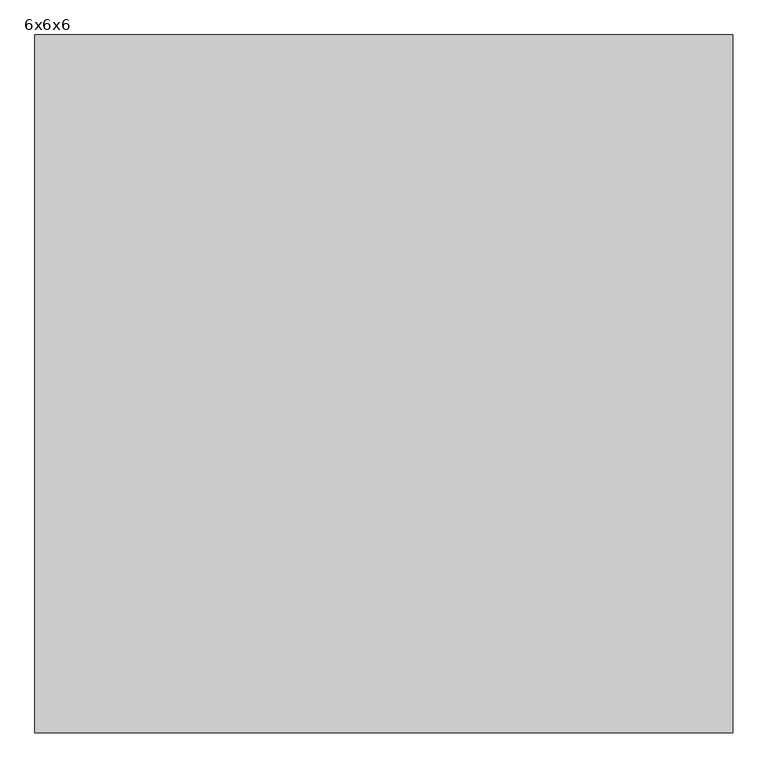
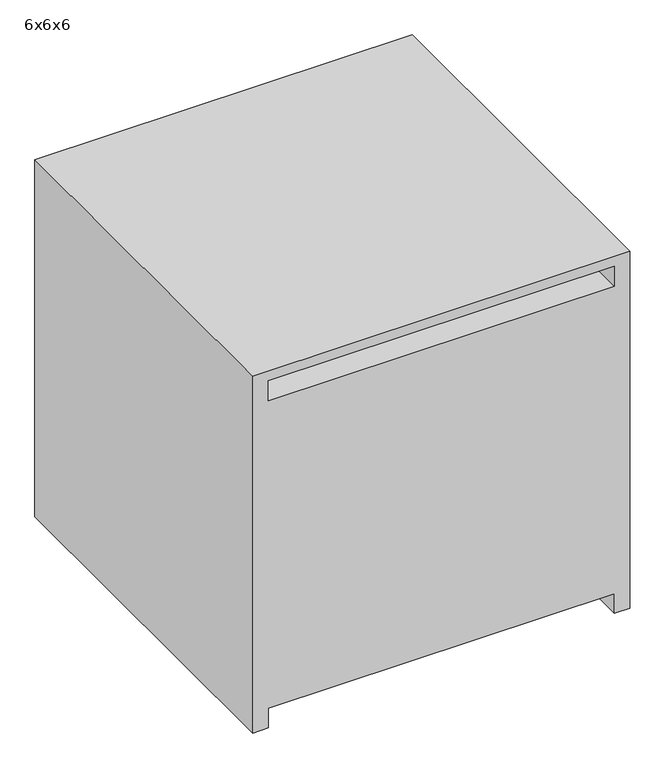
"""IFC4 building model written with IfcOpenShell, lengths in millimetres: proxy geometry, Transformer-Dry-Type-Siemens : 6x6x6."""

import ifcopenshell
import ifcopenshell.guid

model = None  # the IFC model being written
_history = None  # IfcOwnerHistory: only IFC2X3 demands one
_inside = {}  # id of a spatial element -> (the spatial element, [elements in it])
_under = {}  # id of a project, library or spatial element -> (it, [spatial elements below it])
_declared = {}  # id of a project -> (the project, [libraries it declares])
_typed = {}  # id of a type object -> (the type object, [elements of that type])
_made_of = {}  # id of a material, layer set ... -> (it, [elements and type objects made of it])


def new_model(schema):
    """Start an empty IFC model of exactly this schema.

    Asked for "IFC4X3", IfcOpenShell would pick the latest addendum, in which some entities
    have other attributes; the version numbers below select the first issue.
    IFC2X3 requires an IfcOwnerHistory on every rooted entity: one is made here for all.
    """
    global model, _history
    if schema == "IFC4X3":
        model = ifcopenshell.file(schema_version=(4, 3, 0, 0))
    else:
        model = ifcopenshell.file(schema=schema)
    _inside.clear()
    _under.clear()
    _declared.clear()
    _typed.clear()
    _made_of.clear()
    _history = None
    if model.schema == "IFC2X3":
        org = make("IfcOrganization", Name="unknown")
        user = make(
            "IfcPersonAndOrganization",
            ThePerson=make("IfcPerson", FamilyName="unknown"),
            TheOrganization=org,
        )
        app = make(
            "IfcApplication",
            ApplicationDeveloper=org,
            Version="unknown",
            ApplicationFullName="unknown",
            ApplicationIdentifier="unknown",
        )
        _history = make(
            "IfcOwnerHistory",
            OwningUser=user,
            OwningApplication=app,
            ChangeAction="ADDED",
            CreationDate=0,
        )
    return model


def make(cls, **values):
    """One entity of the class cls with the attributes given. An attribute that is None is left unset."""
    return model.create_entity(
        cls, **{name: value for name, value in values.items() if value is not None}
    )


def rooted(cls, **values):
    """An entity with a GlobalId (a new one), such as an element, a storey or a relation."""
    return make(cls, GlobalId=ifcopenshell.guid.new(), OwnerHistory=_history, **values)


def si_unit(unit_type, name, prefix=None):
    """IfcSIUnit, for example si_unit("LENGTHUNIT", "METRE", prefix="MILLI")."""
    return make("IfcSIUnit", UnitType=unit_type, Prefix=prefix, Name=name)


def assignment(units):
    """IfcUnitAssignment: the units of a project."""
    return None if units is None else make("IfcUnitAssignment", Units=units)


def point(xyz):
    """IfcCartesianPoint."""
    return None if xyz is None else make("IfcCartesianPoint", Coordinates=xyz)


def direction(xyz):
    """IfcDirection."""
    return None if xyz is None else make("IfcDirection", DirectionRatios=xyz)


def frame(location, z_axis=None, x_axis=None):
    """IfcAxis2Placement3D, a coordinate frame: its origin and axes. An axis left out is left unset."""
    return make(
        "IfcAxis2Placement3D",
        Location=point(location),
        Axis=direction(z_axis),
        RefDirection=direction(x_axis),
    )


def origin():
    """The frame at (0, 0, 0) with its axes left unset."""
    return frame((0.0, 0.0, 0.0))


def place(relative_to, where):
    """IfcLocalPlacement: puts the frame where relative to a parent placement (None: the world)."""
    return make(
        "IfcLocalPlacement", PlacementRelTo=relative_to, RelativePlacement=where
    )


def context(
    kind, dimensions, precision=None, world=None, true_north=None, identifier=None
):
    """IfcGeometricRepresentationContext, for example the 3D "Model" context."""
    return make(
        "IfcGeometricRepresentationContext",
        ContextIdentifier=identifier,
        ContextType=kind,
        CoordinateSpaceDimension=dimensions,
        Precision=precision,
        WorldCoordinateSystem=world,
        TrueNorth=true_north,
    )


def project(units=None, contexts=None):
    """IfcProject with its units and contexts."""
    return rooted(
        "IfcProject",
        Name="project",
        RepresentationContexts=contexts,
        UnitsInContext=assignment(units),
    )


def spatial(cls, under=None, at=None, **own):
    """A site, building, storey or space (cls), placed at a placement, below another one or the project."""
    s = rooted(cls, ObjectPlacement=at, **own)
    if under is not None:
        _under.setdefault(under.id(), (under, []))[1].append(s)
    return s


def polyline(points):
    """IfcPolyline through the points."""
    return make("IfcPolyline", Points=[point(p) for p in points])


def outline(outer, holes=None, kind="AREA"):
    """IfcArbitraryClosedProfileDef: a profile drawn as a closed curve; with holes, ...WithVoids."""
    if holes is None:
        return make("IfcArbitraryClosedProfileDef", ProfileType=kind, OuterCurve=outer)
    return make(
        "IfcArbitraryProfileDefWithVoids",
        ProfileType=kind,
        OuterCurve=outer,
        InnerCurves=holes,
    )


def extrude(swept, where, along, depth):
    """IfcExtrudedAreaSolid: the profile swept, set in the frame where, extruded along a direction by depth."""
    return make(
        "IfcExtrudedAreaSolid",
        SweptArea=swept,
        Position=where,
        ExtrudedDirection=direction(along),
        Depth=depth,
    )


def shape(context_of_items, identifier, shape_type, items):
    """IfcShapeRepresentation: the items that make up one representation, for example the "Body"."""
    return make(
        "IfcShapeRepresentation",
        ContextOfItems=context_of_items,
        RepresentationIdentifier=identifier,
        RepresentationType=shape_type,
        Items=items,
    )


def source(mapping_origin, context_of_items, identifier, shape_type, items):
    """IfcRepresentationMap: a shape defined once, which mapped items show again and again."""
    return make(
        "IfcRepresentationMap",
        MappingOrigin=mapping_origin,
        MappedRepresentation=shape(context_of_items, identifier, shape_type, items),
    )


def transform(
    local_origin,
    x_axis=None,
    y_axis=None,
    z_axis=None,
    scale=None,
    scale2=None,
    scale3=None,
    uniform=True,
):
    """IfcCartesianTransformationOperator3D, or its non-uniform kind. x_axis, y_axis, z_axis: its Axis1, 2, 3."""
    if uniform:
        return make(
            "IfcCartesianTransformationOperator3D",
            Axis1=direction(x_axis),
            Axis2=direction(y_axis),
            LocalOrigin=point(local_origin),
            Scale=scale,
            Axis3=direction(z_axis),
        )
    return make(
        "IfcCartesianTransformationOperator3DnonUniform",
        Axis1=direction(x_axis),
        Axis2=direction(y_axis),
        LocalOrigin=point(local_origin),
        Scale=scale,
        Axis3=direction(z_axis),
        Scale2=scale2,
        Scale3=scale3,
    )


def mapped(mapping_source, mapping_target):
    """IfcMappedItem: shows the shape of a source again, moved by a transform."""
    return make(
        "IfcMappedItem", MappingSource=mapping_source, MappingTarget=mapping_target
    )


def made_of(thing, what):
    """Note that an element or type object is made of a material, layer set ...; save() writes the relation."""
    if what is not None:
        _made_of.setdefault(what.id(), (what, []))[1].append(thing)
    return thing


def element(
    cls,
    number,
    at=None,
    inside=None,
    cuts=None,
    type_object=None,
    material=None,
    context=None,
    identifier="Body",
    shape_type=None,
    held_by="IfcProductDefinitionShape",
    body=None,
    shapes=None,
    **own,
):
    """One element of the class cls, such as IfcWall. Its Tag is "e" and its number.

    at: its placement. inside: the storey or other place that contains it. cuts: it is an
    opening in that element (IfcRelVoidsElement). A single representation is given by context,
    identifier, shape_type and body (its items); several are given by shapes. held_by: the class
    of the entity that holds the representations. save() writes the other relations.
    """
    e = rooted(cls, Tag="e%d" % number, ObjectPlacement=at, **own)
    if body is not None:
        shapes = [shape(context, identifier, shape_type, body)]
    if shapes is not None:
        e.Representation = make(held_by, Representations=shapes)
    if inside is not None:
        _inside.setdefault(inside.id(), (inside, []))[1].append(e)
    if cuts is not None:
        rooted(
            "IfcRelVoidsElement", RelatingBuildingElement=cuts, RelatedOpeningElement=e
        )
    if type_object is not None:
        _typed.setdefault(type_object.id(), (type_object, []))[1].append(e)
    return made_of(e, material)


def aggregate(whole, parts):
    """IfcRelAggregates: a whole, such as a stair, and the parts it consists of."""
    return rooted("IfcRelAggregates", RelatingObject=whole, RelatedObjects=parts)


def save(model, path):
    """Write the relations noted so far, then the file.

    IfcRelAggregates (storeys below a building ...), IfcRelContainedInSpatialStructure (elements
    in a storey), IfcRelDefinesByType, IfcRelAssociatesMaterial and IfcRelDeclares: one each for
    every whole, place, type object, material and project.
    """
    for whole, parts in _under.values():
        aggregate(whole, parts)
    for where, things in _inside.values():
        rooted(
            "IfcRelContainedInSpatialStructure",
            RelatedElements=things,
            RelatingStructure=where,
        )
    for kind, things in _typed.values():
        rooted("IfcRelDefinesByType", RelatedObjects=things, RelatingType=kind)
    for what, things in _made_of.values():
        rooted("IfcRelAssociatesMaterial", RelatedObjects=things, RelatingMaterial=what)
    for by, libraries in _declared.values():
        rooted("IfcRelDeclares", RelatingContext=by, RelatedDefinitions=libraries)
    model.write(path)


def proxy_6x6x6_c494abd1(model_context):
    return source(origin(), model_context, "Body", "SweptSolid", [
        extrude(outline(polyline([(1828.8, 914.4), (1828.8, -914.4), (0.0, -914.4), (0.0, -838.2), (101.6, -838.2), (101.6, 838.2), (0.0, 838.2), (0.0, 914.4), (1828.8, 914.4)]), holes=[polyline([(1778.0, 838.2), (1676.4, 838.2), (1676.4, -838.2), (1778.0, -838.2), (1778.0, 838.2)])]), frame((0.0, -914.4, 0.0), z_axis=(0.0, 1.0, 0.0), x_axis=(0.0, 0.0, 1.0)), (0.0, 0.0, 1.0), 1828.8),
    ])


if __name__ == "__main__":
    model = new_model("IFC4")
    model_context = context("Model", 3, world=origin())
    ifc_project = project(units=[si_unit("LENGTHUNIT", "METRE", prefix="MILLI")], contexts=[model_context])
    site = spatial("IfcSite", under=ifc_project)
    building = spatial("IfcBuilding", under=site)
    placement = place(None, origin())
    proxy_6x6x6_shape = proxy_6x6x6_c494abd1(model_context)
    element("IfcBuildingElementProxy", 1, Name="Transformer-Dry-Type-Siemens : 6x6x6", ObjectType="Transformer-Dry-Type-Siemens : 6x6x6", at=placement, inside=building, context=model_context, shape_type="MappedRepresentation", body=[
        mapped(proxy_6x6x6_shape, transform((0.0, 0.0, 0.0), x_axis=(1.0, 0.0, 0.0), y_axis=(0.0, 1.0, 0.0), z_axis=(0.0, 0.0, 1.0))),
    ])
    save(model, "model.ifc")

# Revit data of these elements
# Type "Transformer-Dry-Type-Siemens : 6x6x6"
#   Weight = "5500"
#   Wattage = "DO NOT USE"
#   Voltage = "DO NOT USE"
#   URL = "http://www.usa.siemens.com/ce"
#   Transformer Material = "Aluminum"
#   Product Page URL = "http://www.sea.siemens.com/us/Products/PowerDistribution/Product/Transformers/Pages/Transformers.aspx"
#   Product Documentation Link = "http://www.sea.siemens.com/us/internet-dms/Internet/ConsultingEngineersComm/General/Docs/drytrans.pdf"
#   Model = "3F3Y015K13TP1"
#   Manufacturer = "Siemens Industry"
#   KVA = "750"
#   K Factor = "13"
#   Description = "Transformer"
#   Deg Rise = "150"
#   Copyright © = "© Siemens Industry, Inc. 2011"
#   CTRL Connector Description = "Equipment Power"
#   BOM URL [instance default] = ""
#   Assembly Code = "D5090900"
#   Width = 6' - 0"
#   Primary Voltage = 480 V
#   Power Factor = 1
#   Height = 6' - 0"
#   Depth = 6' - 0"
#   Apparent Load [instance default] = 0 VA
#   Has Not Contacted Siemens For Configuration [instance default] = no
#   Contacted Siemens For Configuration [instance default] = yes
#   Text Material = Paint- Siemens - Dark
#   Frame Material = Metal - Siemens - Steel
# Element 1 (IfcBuildingElementProxy, "Transformer-Dry-Type-Siemens : 6x6x6")
#   Materials on its faces: "Metal - Siemens - Steel"
# Materials
#   "Paint- Siemens - Dark": class "Metal", colour RGB 175 38 68, transparency 0
#   "Metal - Siemens - Steel": class "Metal", colour RGB 63 114 97, transparency 0, Cost = 0
